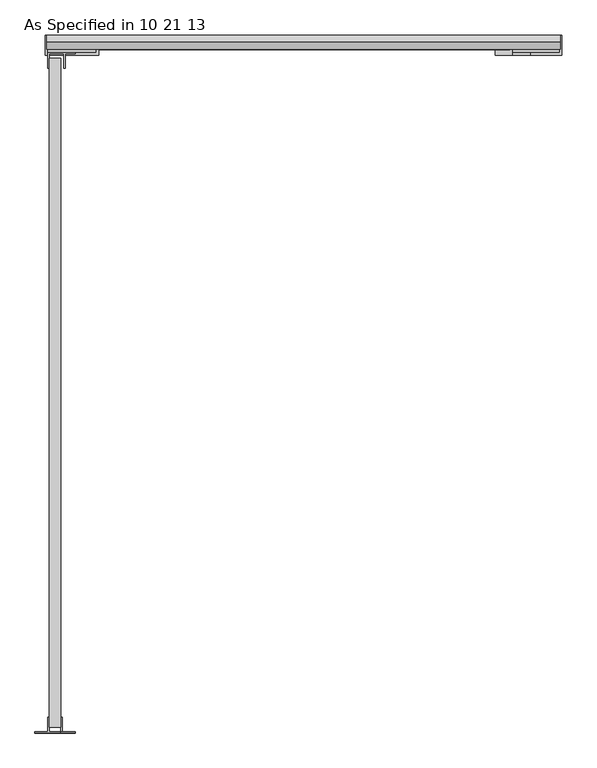
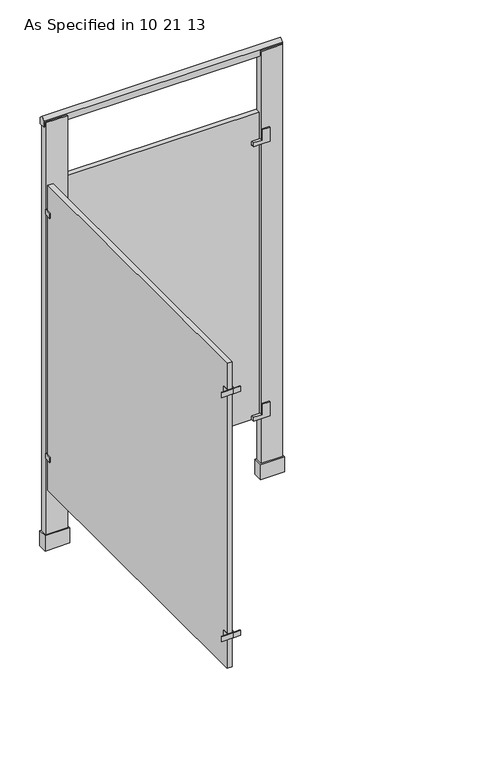
"""IFC4 building model written with IfcOpenShell, lengths in millimetres: proxy geometry, Toilet-Partition_Spec-Rite_Floor-Supported_Headrail : As Specified in 10 21 13."""

from ifc_helpers import new_model, si_unit, frame, origin, origin_with_axes, place, context, project, spatial, polyline, outline, extrude, source, transform, mapped, element, save


def as_specified_in_10_21_13_a0c95563(model_context):
    return source(origin(), model_context, "Body", "SweptSolid", [
        extrude(outline(polyline([(105.4810872, 2316.1677205), (105.4810872, 2284.510976), (102.3060872, 2284.510976), (102.3060872, 2319.3427205), (162.6310872, 2319.3427205), (162.6310872, 2316.2124537), (140.4060872, 2316.2124537), (140.4060872, 2284.510976), (137.2310872, 2284.510976), (137.2310872, 2316.1677205), (105.4810872, 2316.1677205)])), frame((0.0, 0.0, 1676.4), z_axis=(0.0, 0.0, 1.0), x_axis=(1.0, 0.0, 0.0)), (0.0, 0.0, 1.0), 25.4),
        extrude(outline(polyline([(105.4810872, 2316.1677205), (105.4810872, 2284.510976), (102.3060872, 2284.510976), (102.3060872, 2319.3427205), (162.6310872, 2319.3427205), (162.6310872, 2316.2124537), (140.4060872, 2316.2124537), (140.4060872, 2284.510976), (137.2310872, 2284.510976), (137.2310872, 2316.1677205), (105.4810872, 2316.1677205)])), frame((0.0, 0.0, 457.2), z_axis=(0.0, 0.0, 1.0), x_axis=(1.0, 0.0, 0.0)), (0.0, 0.0, 1.0), 25.4),
        extrude(outline(polyline([(162.6310872, 827.0927205), (130.8810872, 827.0927205), (130.8810872, 830.2677205), (162.6310872, 830.2677205), (162.6310872, 827.0927205)])), frame((0.0, 0.0, 1676.4), z_axis=(0.0, 0.0, 1.0), x_axis=(1.0, 0.0, 0.0)), (0.0, 0.0, 1.0), 25.4),
        extrude(outline(polyline([(130.8810872, 830.2677205), (130.8810872, 861.924465), (134.0560872, 861.924465), (134.0560872, 827.0927205), (73.7310872, 827.0927205), (73.7310872, 830.2229872), (102.3060872, 830.2229872), (102.3060872, 861.924465), (105.4810872, 861.924465), (105.4810872, 830.2677205), (130.8810872, 830.2677205)])), frame((0.0, 0.0, 1676.4), z_axis=(0.0, 0.0, 1.0), x_axis=(1.0, 0.0, 0.0)), (0.0, 0.0, 1.0), 25.4),
        extrude(outline(polyline([(162.6310872, 827.0927205), (130.8810872, 827.0927205), (130.8810872, 830.2677205), (162.6310872, 830.2677205), (162.6310872, 827.0927205)])), frame((0.0, 0.0, 457.2), z_axis=(0.0, 0.0, 1.0), x_axis=(1.0, 0.0, 0.0)), (0.0, 0.0, 1.0), 25.4),
        extrude(outline(polyline([(130.8810872, 830.2677205), (130.8810872, 861.924465), (134.0560872, 861.924465), (134.0560872, 827.0927205), (73.7310872, 827.0927205), (73.7310872, 830.2229872), (102.3060872, 830.2229872), (102.3060872, 861.924465), (105.4810872, 861.924465), (105.4810872, 830.2677205), (130.8810872, 830.2677205)])), frame((0.0, 0.0, 457.2), z_axis=(0.0, 0.0, 1.0), x_axis=(1.0, 0.0, 0.0)), (0.0, 0.0, 1.0), 25.4),
        extrude(outline(polyline([(130.8810872, 839.7927205), (105.4810872, 839.7927205), (105.4810872, 2306.6427205), (130.8810872, 2306.6427205), (130.8810872, 839.7927205)])), frame((0.0, 0.0, 304.8), z_axis=(0.0, 0.0, 1.0), x_axis=(1.0, 0.0, 0.0)), (0.0, 0.0, 1.0), 1524.0),
        extrude(outline(polyline([(1223.0810872, 2351.0927205), (1223.0810872, 2319.3427205), (1121.4810872, 2319.3427205), (1121.4810872, 2351.0927205), (1223.0810872, 2351.0927205)])), origin_with_axes(), (0.0, 0.0, 1.0), 2133.6),
        extrude(outline(polyline([(207.0810872, 2351.0927205), (207.0810872, 2319.3427205), (102.3060872, 2319.3427205), (102.3060872, 2351.0927205), (207.0810872, 2351.0927205)])), origin_with_axes(), (0.0, 0.0, 1.0), 2133.6),
        extrude(outline(polyline([(168.9810872, 2357.4427205), (232.4810872, 2357.4427205), (232.4810872, 2351.0927205), (168.9810872, 2351.0927205), (168.9810872, 2357.4427205)])), frame((0.0, 0.0, 1015.4167184), z_axis=(0.0, 0.0, 1.0), x_axis=(1.0, 0.0, 0.0)), (0.0, 0.0, 1.0), 51.9665631),
        extrude(outline(polyline([(374.65, 1159.5810872), (374.65, 1121.4810872), (323.85, 1121.4810872), (323.85, 1083.3810872), (304.8, 1083.3810872), (304.8, 1159.5810872), (374.65, 1159.5810872)])), frame((0.0, 2313.0069356, 0.0), z_axis=(0.0, 1.0, 0.0), x_axis=(0.0, 0.0, 1.0)), (0.0, 0.0, 1.0), 44.4357849),
        extrude(outline(polyline([(1746.25, 1159.5810872), (1746.25, 1121.4810872), (1695.45, 1121.4810872), (1695.45, 1083.3810872), (1676.4, 1083.3810872), (1676.4, 1121.4810872), (1676.4, 1159.5810872), (1746.25, 1159.5810872)])), frame((0.0, 2313.0069356, 0.0), z_axis=(0.0, 1.0, 0.0), x_axis=(0.0, 0.0, 1.0)), (0.0, 0.0, 1.0), 44.4357849),
        extrude(outline(polyline([(304.8, 213.4310872), (304.8, 1077.0310872), (323.85, 1077.0310872), (323.85, 1115.1310872), (1674.426485, 1115.1310872), (1674.426485, 1077.0310872), (1695.45, 1077.0310872), (1695.45, 1115.1310872), (1828.8, 1115.1310872), (1828.8, 213.4310872), (304.8, 213.4310872)])), frame((0.0, 2325.6927205, 0.0), z_axis=(0.0, 1.0, 0.0), x_axis=(0.0, 0.0, 1.0)), (0.0, 0.0, 1.0), 25.4),
        extrude(outline(polyline([(2357.4427205, 2139.95), (2357.4427205, 2108.2), (2325.6927205, 2108.2), (2325.6927205, 2139.95), (2341.5677205, 2155.825), (2357.4427205, 2139.95)])), frame((99.7568731, 0.0, 0.0), z_axis=(1.0, 0.0, 0.0), x_axis=(0.0, 1.0, 0.0)), (0.0, 0.0, 1.0), 1126.0239485),
        extrude(outline(polyline([(1115.1310872, 2357.6771735), (1229.4310872, 2357.6771735), (1229.4310872, 2313.0069356), (1115.1310872, 2313.0069356), (1115.1310872, 2357.6771735)])), origin_with_axes(), (0.0, 0.0, 1.0), 76.2),
        extrude(outline(polyline([(95.9560872, 2357.317106), (213.4310872, 2357.317106), (213.4310872, 2313.0516689), (95.9560872, 2313.0516689), (95.9560872, 2357.317106)])), origin_with_axes(), (0.0, 0.0, 1.0), 76.2),
    ])


if __name__ == "__main__":
    model = new_model("IFC4")
    model_context = context("Model", 3, world=origin())
    ifc_project = project(units=[si_unit("LENGTHUNIT", "METRE", prefix="MILLI")], contexts=[model_context])
    site = spatial("IfcSite", under=ifc_project)
    building = spatial("IfcBuilding", under=site)
    placement = place(None, origin())
    as_specified_in_10_21_13_shape = as_specified_in_10_21_13_a0c95563(model_context)
    element("IfcBuildingElementProxy", 1, Name="Toilet-Partition_Spec-Rite_Floor-Supported_Headrail : As Specified in 10 21 13", ObjectType="Toilet-Partition_Spec-Rite_Floor-Supported_Headrail : As Specified in 10 21 13", at=placement, inside=building, context=model_context, shape_type="MappedRepresentation", body=[
        mapped(as_specified_in_10_21_13_shape, transform((0.0, 0.0, 0.0), x_axis=(1.0, 0.0, 0.0), y_axis=(0.0, 1.0, 0.0), z_axis=(0.0, 0.0, 1.0))),
    ])
    save(model, "model.ifc")

# Revit data of these elements
# Type "Toilet-Partition_Spec-Rite_Floor-Supported_Headrail : As Specified in 10 21 13"
#   URL = "http://www.specritedesigns.com/"
#   UL Fire Rating [instance default] = ""
#   Manufacturer Phone - Toll Free = "877-249-6864"
#   Installation-Fabrication = "http://www.specritedesigns.com/partition_systems.aspx"
#   Green Building-LEED = "http://www.arcat.com/green/clients/leed_data_43944.html"
#   Specification = "http://www.arcat.com/sdspecs/htm/10150you.htm"
#   Send Message = "http://www.arcat.com/users.pl?action=UserEmail&company=Spec-Rite%20Designs%20LLC&coid=43944&rep=146&fax=314-771-4597&mf="
#   Sales Information = "http://www.specritedesigns.com/local_rep.aspx"
#   Revision = "R1_04/2010"
#   Product Properties = "http://www.arcat.com/bim/bim_info.pl?fn=Toilet-Partition_Spec-Rite_"
#   Product Data = "http://www.arcat.com/arcatcos/cos43/arc43944.html"
#   Model = "As Specified in 10 21 13"
#   Manufacturer's Notes = ""
#   Manufacturer Website = "http://www.specritedesigns.com/"
#   Manufacturer Phone = ""
#   Manufacturer Fax = "314-771-4597"
#   Manufacturer Address = "1054 Central Industrial Dr.; St. Louis; MO 63110"
#   Manufacturer = "Spec-Rite Designs LLC"
#   Keynote = "10 21 13"
#   Installation Phase = ""
#   Drawn By = "Robert S. Weygant, CSI, CDT, SCIP"
#   Core Material [instance default] = ""
#   Copyright = "2010, ARCAT, Inc."
#   Description = "As Specified in 10 21 13"
#   Construction Details = "http://www.specritedesigns.com/LinkClick.aspx?fileticket=c2fn%2bPpDPB4%3d&tabid=106"
#   Assembly Code = "C1010400"
#   topoffset = 0' - 0 1/4"
#   hngpnlconstrain [instance default] = 0' - 5 1/8"
#   hngpnl2 [instance default] = 0' - 1 1/8"
#   capoffset = 0' - 0 1/4"
#   Stile Thickness = 0' - 1 1/4"
#   Stall Width = 3' - 7"
#   Stall Depth = 5' - 0"
#   Pilaster Height = 7' - 0"
#   Panel Thickness = 0' - 1"
#   Panel Height = 5' - 0"
#   Front Panel Width_Strike Side = 0' - 3"
#   Reveal Clearance = 0' - 0 1/2"
#   Front Panel Width_Hinge Side = 0' - 4"
#   Door Width = 3' - 0"
#   Door Thickness = 0' - 1"
#   Distance from Floor to Panel = 1' - 0"
#   strkhdwr [instance default] = no
#   Warranty Duration (Years) = 0
#   Terminates at Wall_Strike Side [instance default] = no
#   Terminates at Wall_Hinge Side [instance default] = no
#   Return Rail - Strike Side [instance default] = yes
#   Return Rail - Hinge Side [instance default] = yes
#   Outswing [instance default] = no
#   Inswing [instance default] = yes
#   End Panel_Strike Side [instance default] = yes
#   Maintenance Schedule (Months) = 0
#   End Panel_Hinge Side [instance default] = yes
#   Expected Lifespan (Years) = 0
#   Brackets_Vertical = 2
#   Headrail Material = Aluminum - Extruded - Satin Anodized Finish
#   Hardware Type [instance default] = element 529356
#   Panel Material [instance default] = Phenolic Core - Color as Specified
#   Hardware Finish [instance default] = Stainless Steel - Type 304 #4 Brushed Finish
#   Type Comments = ""
# Element 1 (IfcBuildingElementProxy, "Toilet-Partition_Spec-Rite_Floor-Supported_Headrail : As Specified in 10 21 13")
#   hngpnlconstrain = 0' - 4"
#   Return Rail - Strike Side = no
#   Return Rail - Hinge Side = no
#   Outswing = yes
#   Inswing = no
#   End Panel_Hinge Side = no
#   Materials on its faces: "Stainless Steel - Type 304 #4 Brushed Finish", "Phenolic Core - Color as Specified", "Aluminum - Extruded - Satin Anodized Finish"
# Materials
#   "Aluminum - Extruded - Satin Anodized Finish": class "Hardware Finishes", colour RGB 244 244 244, transparency 0, Model = "Aluminum - Extruded - Satin Anodized Finish", Description = "Aluminum - Extruded - Satin Anodized Finish", Cost = 0
#   "Phenolic Core - Color as Specified": class "Spec-Rite Partition Finishes", colour RGB 215 199 171, transparency 0, Keynote = "10 21 00", Model = "Phenolic Core - Color as Specified in 10 21 00", Manufacturer = "Spec-Rite Designs LLC", URL = "http://www.specritedesigns.com/", Description = "Phenolic Core - Color as Specified in 10 21 00", Cost = 0
#   "Stainless Steel - Type 304 #4 Brushed Finish": class "Hardware Finishes", colour RGB 189 187 185, transparency 0, Model = "Stainless Steel - Type 304 #4 Brushed Finish", Description = "Stainless Steel - Type 304 #4 Brushed Finish", Cost = 0
